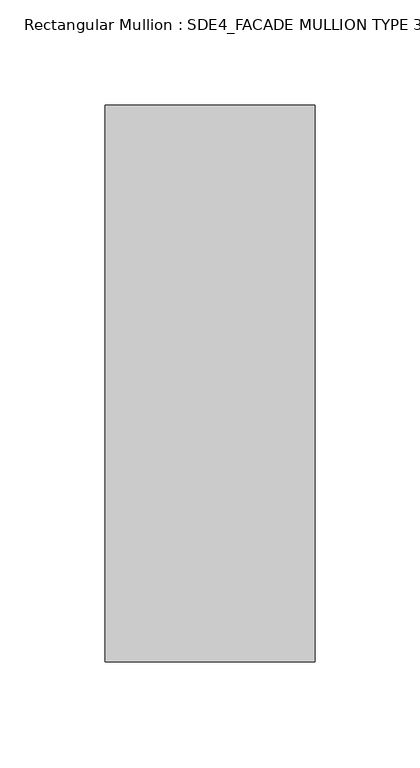
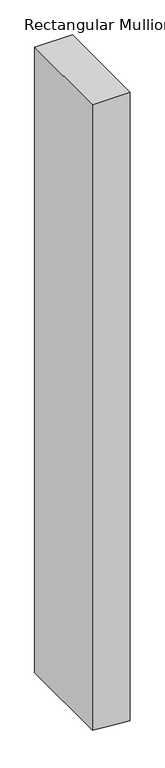
"""IFC4 building model written with IfcOpenShell, lengths in millimetres: member geometry, Rectangular Mullion : SDE4_FACADE MULLION TYPE 3."""

from ifc_helpers import new_model, si_unit, frame, origin, place, context, project, spatial, polyline, outline, extrude, source, transform, mapped, element, save


def rectangular_mullion_sde4_facade_mullion_type_3_a5cafc9c(model_context):
    return source(origin(), model_context, "Body", "SweptSolid", [
        extrude(outline(polyline([(0.0, 50.0), (0.0, -50.0), (-1751.9724847, -50.0), (-1756.0385637, 3.056508), (-1759.636161, 50.0), (0.0, 50.0)])), frame((0.0, -132.5, 0.0), z_axis=(0.0, 1.0, 0.0), x_axis=(0.0, 0.0, 1.0)), (0.0, 0.0, 1.0), 265.0),
    ])


if __name__ == "__main__":
    model = new_model("IFC4")
    model_context = context("Model", 3, world=origin())
    ifc_project = project(units=[si_unit("LENGTHUNIT", "METRE", prefix="MILLI")], contexts=[model_context])
    site = spatial("IfcSite", under=ifc_project)
    building = spatial("IfcBuilding", under=site)
    placement = place(None, origin())
    rectangular_mullion_sde4_facade_mullion_type_3_shape = rectangular_mullion_sde4_facade_mullion_type_3_a5cafc9c(model_context)
    element("IfcMember", 1, ObjectType="Rectangular Mullion : SDE4_FACADE MULLION TYPE 3", at=placement, inside=building, context=model_context, shape_type="MappedRepresentation", body=[
        mapped(rectangular_mullion_sde4_facade_mullion_type_3_shape, transform((0.0, 0.0, 0.0), x_axis=(1.0, 0.0, 0.0), y_axis=(0.0, 1.0, 0.0), z_axis=(0.0, 0.0, 1.0))),
    ])
    save(model, "model.ifc")

# Revit data of these elements
# Type "Rectangular Mullion : SDE4_FACADE MULLION TYPE 3"
#   built-in parameter 1007322 = 0.869423 (stored number, unit not read)
#   built-in parameter 1007321 = 0.164042 (stored number, unit not read)
#   built-in parameter 1007320 = 0.164042 (stored number, unit not read)
